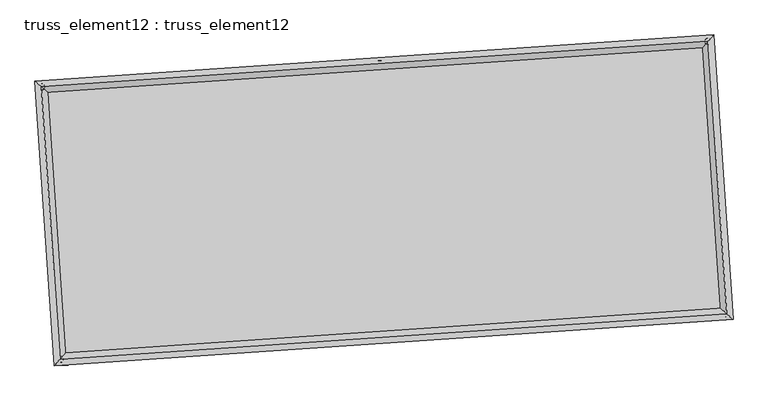
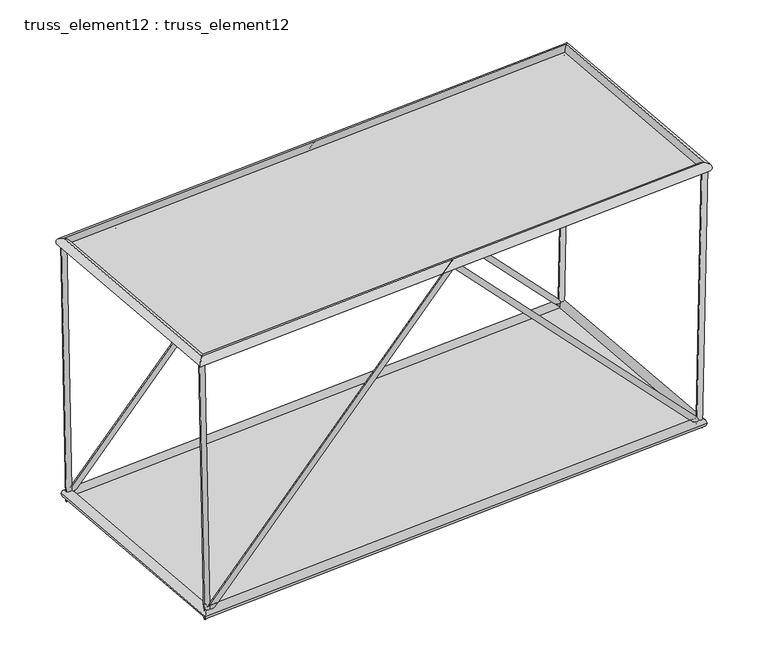
"""IFC4 building model written with IfcOpenShell, lengths in millimetres: plate geometry, truss_element12 : truss_element12."""

import ifcopenshell
import ifcopenshell.guid

model = None  # the IFC model being written
_history = None  # IfcOwnerHistory: only IFC2X3 demands one
_inside = {}  # id of a spatial element -> (the spatial element, [elements in it])
_under = {}  # id of a project, library or spatial element -> (it, [spatial elements below it])
_declared = {}  # id of a project -> (the project, [libraries it declares])
_typed = {}  # id of a type object -> (the type object, [elements of that type])
_made_of = {}  # id of a material, layer set ... -> (it, [elements and type objects made of it])


def new_model(schema):
    """Start an empty IFC model of exactly this schema.

    Asked for "IFC4X3", IfcOpenShell would pick the latest addendum, in which some entities
    have other attributes; the version numbers below select the first issue.
    IFC2X3 requires an IfcOwnerHistory on every rooted entity: one is made here for all.
    """
    global model, _history
    if schema == "IFC4X3":
        model = ifcopenshell.file(schema_version=(4, 3, 0, 0))
    else:
        model = ifcopenshell.file(schema=schema)
    _inside.clear()
    _under.clear()
    _declared.clear()
    _typed.clear()
    _made_of.clear()
    _history = None
    if model.schema == "IFC2X3":
        org = make("IfcOrganization", Name="unknown")
        user = make(
            "IfcPersonAndOrganization",
            ThePerson=make("IfcPerson", FamilyName="unknown"),
            TheOrganization=org,
        )
        app = make(
            "IfcApplication",
            ApplicationDeveloper=org,
            Version="unknown",
            ApplicationFullName="unknown",
            ApplicationIdentifier="unknown",
        )
        _history = make(
            "IfcOwnerHistory",
            OwningUser=user,
            OwningApplication=app,
            ChangeAction="ADDED",
            CreationDate=0,
        )
    return model


def make(cls, **values):
    """One entity of the class cls with the attributes given. An attribute that is None is left unset."""
    return model.create_entity(
        cls, **{name: value for name, value in values.items() if value is not None}
    )


def rooted(cls, **values):
    """An entity with a GlobalId (a new one), such as an element, a storey or a relation."""
    return make(cls, GlobalId=ifcopenshell.guid.new(), OwnerHistory=_history, **values)


def si_unit(unit_type, name, prefix=None):
    """IfcSIUnit, for example si_unit("LENGTHUNIT", "METRE", prefix="MILLI")."""
    return make("IfcSIUnit", UnitType=unit_type, Prefix=prefix, Name=name)


def assignment(units):
    """IfcUnitAssignment: the units of a project."""
    return None if units is None else make("IfcUnitAssignment", Units=units)


def point(xyz):
    """IfcCartesianPoint."""
    return None if xyz is None else make("IfcCartesianPoint", Coordinates=xyz)


def direction(xyz):
    """IfcDirection."""
    return None if xyz is None else make("IfcDirection", DirectionRatios=xyz)


def frame(location, z_axis=None, x_axis=None):
    """IfcAxis2Placement3D, a coordinate frame: its origin and axes. An axis left out is left unset."""
    return make(
        "IfcAxis2Placement3D",
        Location=point(location),
        Axis=direction(z_axis),
        RefDirection=direction(x_axis),
    )


def origin():
    """The frame at (0, 0, 0) with its axes left unset."""
    return frame((0.0, 0.0, 0.0))


def origin_with_axes():
    """The frame at (0, 0, 0) with the z axis (0, 0, 1) and the x axis (1, 0, 0) written out."""
    return frame((0.0, 0.0, 0.0), z_axis=(0.0, 0.0, 1.0), x_axis=(1.0, 0.0, 0.0))


def place(relative_to, where):
    """IfcLocalPlacement: puts the frame where relative to a parent placement (None: the world)."""
    return make(
        "IfcLocalPlacement", PlacementRelTo=relative_to, RelativePlacement=where
    )


def context(
    kind, dimensions, precision=None, world=None, true_north=None, identifier=None
):
    """IfcGeometricRepresentationContext, for example the 3D "Model" context."""
    return make(
        "IfcGeometricRepresentationContext",
        ContextIdentifier=identifier,
        ContextType=kind,
        CoordinateSpaceDimension=dimensions,
        Precision=precision,
        WorldCoordinateSystem=world,
        TrueNorth=true_north,
    )


def project(units=None, contexts=None):
    """IfcProject with its units and contexts."""
    return rooted(
        "IfcProject",
        Name="project",
        RepresentationContexts=contexts,
        UnitsInContext=assignment(units),
    )


def spatial(cls, under=None, at=None, **own):
    """A site, building, storey or space (cls), placed at a placement, below another one or the project."""
    s = rooted(cls, ObjectPlacement=at, **own)
    if under is not None:
        _under.setdefault(under.id(), (under, []))[1].append(s)
    return s


def polyline(points):
    """IfcPolyline through the points."""
    return make("IfcPolyline", Points=[point(p) for p in points])


def circle_curve(where, radius):
    """IfcCircle in the frame where."""
    return make("IfcCircle", Position=where, Radius=radius)


def ellipse_curve(where, semi_axis1, semi_axis2):
    """IfcEllipse in the frame where."""
    return make(
        "IfcEllipse", Position=where, SemiAxis1=semi_axis1, SemiAxis2=semi_axis2
    )


def outline(outer, holes=None, kind="AREA"):
    """IfcArbitraryClosedProfileDef: a profile drawn as a closed curve; with holes, ...WithVoids."""
    if holes is None:
        return make("IfcArbitraryClosedProfileDef", ProfileType=kind, OuterCurve=outer)
    return make(
        "IfcArbitraryProfileDefWithVoids",
        ProfileType=kind,
        OuterCurve=outer,
        InnerCurves=holes,
    )


def extrude(swept, where, along, depth):
    """IfcExtrudedAreaSolid: the profile swept, set in the frame where, extruded along a direction by depth."""
    return make(
        "IfcExtrudedAreaSolid",
        SweptArea=swept,
        Position=where,
        ExtrudedDirection=direction(along),
        Depth=depth,
    )


def shape(context_of_items, identifier, shape_type, items):
    """IfcShapeRepresentation: the items that make up one representation, for example the "Body"."""
    return make(
        "IfcShapeRepresentation",
        ContextOfItems=context_of_items,
        RepresentationIdentifier=identifier,
        RepresentationType=shape_type,
        Items=items,
    )


def source(mapping_origin, context_of_items, identifier, shape_type, items):
    """IfcRepresentationMap: a shape defined once, which mapped items show again and again."""
    return make(
        "IfcRepresentationMap",
        MappingOrigin=mapping_origin,
        MappedRepresentation=shape(context_of_items, identifier, shape_type, items),
    )


def transform(
    local_origin,
    x_axis=None,
    y_axis=None,
    z_axis=None,
    scale=None,
    scale2=None,
    scale3=None,
    uniform=True,
):
    """IfcCartesianTransformationOperator3D, or its non-uniform kind. x_axis, y_axis, z_axis: its Axis1, 2, 3."""
    if uniform:
        return make(
            "IfcCartesianTransformationOperator3D",
            Axis1=direction(x_axis),
            Axis2=direction(y_axis),
            LocalOrigin=point(local_origin),
            Scale=scale,
            Axis3=direction(z_axis),
        )
    return make(
        "IfcCartesianTransformationOperator3DnonUniform",
        Axis1=direction(x_axis),
        Axis2=direction(y_axis),
        LocalOrigin=point(local_origin),
        Scale=scale,
        Axis3=direction(z_axis),
        Scale2=scale2,
        Scale3=scale3,
    )


def mapped(mapping_source, mapping_target):
    """IfcMappedItem: shows the shape of a source again, moved by a transform."""
    return make(
        "IfcMappedItem", MappingSource=mapping_source, MappingTarget=mapping_target
    )


def made_of(thing, what):
    """Note that an element or type object is made of a material, layer set ...; save() writes the relation."""
    if what is not None:
        _made_of.setdefault(what.id(), (what, []))[1].append(thing)
    return thing


def element(
    cls,
    number,
    at=None,
    inside=None,
    cuts=None,
    type_object=None,
    material=None,
    context=None,
    identifier="Body",
    shape_type=None,
    held_by="IfcProductDefinitionShape",
    body=None,
    shapes=None,
    **own,
):
    """One element of the class cls, such as IfcWall. Its Tag is "e" and its number.

    at: its placement. inside: the storey or other place that contains it. cuts: it is an
    opening in that element (IfcRelVoidsElement). A single representation is given by context,
    identifier, shape_type and body (its items); several are given by shapes. held_by: the class
    of the entity that holds the representations. save() writes the other relations.
    """
    e = rooted(cls, Tag="e%d" % number, ObjectPlacement=at, **own)
    if body is not None:
        shapes = [shape(context, identifier, shape_type, body)]
    if shapes is not None:
        e.Representation = make(held_by, Representations=shapes)
    if inside is not None:
        _inside.setdefault(inside.id(), (inside, []))[1].append(e)
    if cuts is not None:
        rooted(
            "IfcRelVoidsElement", RelatingBuildingElement=cuts, RelatedOpeningElement=e
        )
    if type_object is not None:
        _typed.setdefault(type_object.id(), (type_object, []))[1].append(e)
    return made_of(e, material)


def aggregate(whole, parts):
    """IfcRelAggregates: a whole, such as a stair, and the parts it consists of."""
    return rooted("IfcRelAggregates", RelatingObject=whole, RelatedObjects=parts)


def save(model, path):
    """Write the relations noted so far, then the file.

    IfcRelAggregates (storeys below a building ...), IfcRelContainedInSpatialStructure (elements
    in a storey), IfcRelDefinesByType, IfcRelAssociatesMaterial and IfcRelDeclares: one each for
    every whole, place, type object, material and project.
    """
    for whole, parts in _under.values():
        aggregate(whole, parts)
    for where, things in _inside.values():
        rooted(
            "IfcRelContainedInSpatialStructure",
            RelatedElements=things,
            RelatingStructure=where,
        )
    for kind, things in _typed.values():
        rooted("IfcRelDefinesByType", RelatedObjects=things, RelatingType=kind)
    for what, things in _made_of.values():
        rooted("IfcRelAssociatesMaterial", RelatedObjects=things, RelatingMaterial=what)
    for by, libraries in _declared.values():
        rooted("IfcRelDeclares", RelatingContext=by, RelatedDefinitions=libraries)
    model.write(path)


def plane_surface(at):
    """IfcPlane: the flat surface through the origin of the frame at, square to its z axis."""
    return make("IfcPlane", Position=at)


def cylinder_surface(at, radius):
    """IfcCylindricalSurface: all points at the distance radius from the z axis of the frame at."""
    return make("IfcCylindricalSurface", Position=at, Radius=radius)


def advanced_brep(points, edges, surfaces, faces):
    """IfcAdvancedBrep: a solid bounded by faces that lie on surfaces and meet in shared edges.

    An edge is (start, end): straight between two places in points (the first is 0);
    or (start, end, curve); or (start, end, curve, False) where it runs against its curve.
    A face is (place in surfaces, loops), or (place, loops, False) where it looks against
    its surface's normal. A loop lists edges by number (the first is 1), with a minus sign
    where the edge is run from its end to its start. The first loop is the outer one.
    """
    corners = [point(p) for p in points]
    vertices = [make("IfcVertexPoint", VertexGeometry=c) for c in corners]
    made = []
    for start, end, *more in edges:
        made.append(
            make(
                "IfcEdgeCurve",
                EdgeStart=vertices[start],
                EdgeEnd=vertices[end],
                EdgeGeometry=more[0] if more else make("IfcPolyline", Points=[corners[start], corners[end]]),
                SameSense=more[1] if len(more) > 1 else True,
            )
        )
    hull = []
    for where, loops, *sense in faces:
        bounds = []
        for j, loop in enumerate(loops):
            ring = [make("IfcOrientedEdge", EdgeElement=made[abs(k) - 1], Orientation=k > 0) for k in loop]
            bounds.append(
                make(
                    "IfcFaceOuterBound" if j == 0 else "IfcFaceBound",
                    Bound=make("IfcEdgeLoop", EdgeList=ring),
                    Orientation=True,
                )
            )
        hull.append(make("IfcAdvancedFace", Bounds=bounds, FaceSurface=surfaces[where], SameSense=sense[0] if sense else True))
    return make("IfcAdvancedBrep", Outer=make("IfcClosedShell", CfsFaces=hull))


def truss_element12_truss_element12_2df4d8d8(model_context):
    return source(origin(), model_context, "Body", "SolidModel", [
        advanced_brep(
        [(-3764.5300605, 2269.433423, 4999.9996325), (-3863.6135877, 2256.0735143, 4998.0077777), (-3667.3556051, 2276.0593798, 121.6771544), (-3761.6312777, 2263.0273003, -121.6771544), (1063.0371685, 2598.6068811, 5071.1337274), (1063.495558, 2592.0343572, 4926.9006014), (5794.7619233, 2921.2452051, 121.686477), (5889.9990537, 2921.1352834, -121.686477), (5890.6143162, 2927.7810154, 5000.0130059), (5990.5947849, 2927.9945239, 4998.0482415)],
        [
            (0, 1, circle_curve(frame((-3814.0718241, 2262.7534687, 4999.0037051), z_axis=(-0.019915676532372622, -0.001357974276168432, 0.9998007410149901), x_axis=(-0.13359951548632418, 0.9910345300462156, -0.001315187399616253)), 50.0)),
            (1, 0, circle_curve(frame((-3814.0718241, 2262.7534687, 4999.0037051), z_axis=(-0.019915676532372622, -0.001357974276168432, 0.9998007410149901), x_axis=(-0.13359951548632418, 0.9910345300462156, -0.001315187399616253)), 50.0)),
            (0, 2),
            (2, 3, ellipse_curve(frame((-3714.4934414, 2269.54334, 0.0), z_axis=(-0.9294501915680613, -0.06337567539207484, 0.36346370542695533), x_axis=(0.36262170398032334, 0.024725795540271416, 0.9316083591495449)), 130.8941732, 50.0)),
            (3, 1),
            (3, 2, ellipse_curve(frame((-3714.4934414, 2269.54334, 0.0), z_axis=(-0.9294501915680613, -0.06337567539207484, 0.36346370542695533), x_axis=(0.36262170398032334, 0.024725795540271416, 0.9316083591495449)), 130.8941732, 50.0)),
            (2, 4),
            (4, 5, ellipse_curve(frame((1063.2663632, 2595.3206192, 4999.0171644), z_axis=(-0.9976833935750009, -0.06802823805824446, -7.079096398268556e-05), x_axis=(7.062696935752604e-05, 4.815784562388573e-06, -0.9999999974943197)), 72.2735967, 50.0)),
            (5, 3),
            (5, 4, ellipse_curve(frame((1063.2663632, 2595.3206192, 4999.0171644), z_axis=(-0.9976833935750009, -0.06802823805824446, -7.079096398268556e-05), x_axis=(7.062696935752604e-05, 4.815784562388573e-06, -0.9999999974943197)), 72.2735967, 50.0)),
            (4, 6),
            (6, 7, ellipse_curve(frame((5842.3804885, 2921.1902443, 0.0), z_axis=(-0.929375267082314, -0.06337056657620659, -0.36365613459350316), x_axis=(-0.3628136873647087, -0.024738886157455623, 0.9315332606904125)), 130.9147553, 50.0)),
            (7, 5),
            (7, 6, ellipse_curve(frame((5842.3804885, 2921.1902443, 0.0), z_axis=(-0.929375267082314, -0.06337056657620659, -0.36365613459350316), x_axis=(-0.3628136873647087, -0.024738886157455623, 0.9315332606904125)), 130.9147553, 50.0)),
            (8, 9, circle_curve(frame((5940.6045505, 2927.8877697, 4999.0306237), z_axis=(0.019644812406203346, 0.0013395050810558434, 0.9998061247420236), x_axis=(-0.0021609883682618125, 0.9999968235657783, -0.001297300129496852)), 50.0)),
            (9, 8, circle_curve(frame((5940.6045505, 2927.8877697, 4999.0306237), z_axis=(0.019644812406203346, 0.0013395050810558434, 0.9998061247420236), x_axis=(-0.0021609883682618125, 0.9999968235657783, -0.001297300129496852)), 50.0)),
            (6, 8),
            (9, 7),
        ],
        [
            plane_surface(frame((-3814.0718241, 2312.7534225, 4999.0716173), z_axis=(-0.019915676532371102, -0.001357974276169366, 0.9998007410149901), x_axis=(0.9998016632453949, -2.7050341500078914e-05, 0.01991565816188513))),
            cylinder_surface(frame((-3814.0718241, 2262.7534687, 4999.0037051), z_axis=(-0.019915676532372622, -0.001357974276168432, 0.9998007410149901), x_axis=(-0.13359951548632418, 0.9910345300462156, -0.001315187399616253)), 50.0),
            cylinder_surface(frame((-3714.4934414, 2269.54334, 0.0), z_axis=(-0.6901619145465996, -0.04705951740188029, -0.7221232121537671), x_axis=(-0.020413692768052043, 0.9987522410377818, -0.045576772259345893)), 50.0),
            cylinder_surface(frame((1063.2663632, 2595.3206192, 4999.0171644), z_axis=(-0.6902639103769979, -0.04706647210983291, 0.722025263570597), x_axis=(-0.11534072659634662, 0.9922795274524686, -0.0455835078392663)), 50.0),
            plane_surface(frame((5940.6045505, 2877.8878145, 4999.0976119), z_axis=(0.01964481240620162, 0.001339505081055023, 0.9998061247420239), x_axis=(0.9998070220525186, -2.631940509978392e-05, -0.0196447947753029))),
            cylinder_surface(frame((5842.3804885, 2921.1902443, 0.0), z_axis=(-0.01964481240620335, -0.0013395050810558436, -0.9998061247420238), x_axis=(-0.0021609883682618125, 0.9999968235657783, -0.001297300129496852)), 50.0),
        ],
        [
            (0, [[1, 2]]),
            (1, [[-1, 3, 4, 5]]),
            (1, [[-2, -5, 6, -3]]),
            (2, [[-4, 7, 8, 9]]),
            (2, [[-6, -9, 10, -7]]),
            (3, [[-8, 11, 12, 13]]),
            (3, [[-10, -13, 14, -11]]),
            (4, [[15, 16]]),
            (5, [[-12, 17, -16, 18]]),
            (5, [[-14, -18, -15, -17]]),
        ],
    ),
        advanced_brep(
        [(-3492.4171076, -1721.3001613, 4999.9996325), (-3591.5006347, -1734.66007, 4998.0077777), (-3395.2426522, -1714.6742045, 121.6771544), (-3489.5183248, -1727.706284, -121.6771544), (1335.1501214, -1392.1267032, 5071.1337274), (1335.6085109, -1398.6992271, 4926.9006014), (6066.8748762, -1069.4883792, 121.686477), (6162.1120066, -1069.5983009, -121.686477), (6162.7272691, -1062.9525689, 5000.0130059), (6262.7077378, -1062.7390604, 4998.0482415)],
        [
            (0, 1, circle_curve(frame((-3541.9588712, -1727.9801156, 4999.0037051), z_axis=(-0.019915676532372775, -0.001357974276168436, 0.9998007410149901), x_axis=(-0.13359951548632507, 0.9910345300462154, -0.001315187399616287)), 50.0)),
            (1, 0, circle_curve(frame((-3541.9588712, -1727.9801156, 4999.0037051), z_axis=(-0.019915676532372775, -0.001357974276168436, 0.9998007410149901), x_axis=(-0.13359951548632507, 0.9910345300462154, -0.001315187399616287)), 50.0)),
            (0, 2),
            (2, 3, ellipse_curve(frame((-3442.3804885, -1721.1902443, 0.0), z_axis=(-0.9294501915680613, -0.06337567539207523, 0.36346370542695516), x_axis=(0.3626217039803232, 0.024725795540271572, 0.9316083591495451)), 130.8941732, 50.0)),
            (3, 1),
            (3, 2, ellipse_curve(frame((-3442.3804885, -1721.1902443, 0.0), z_axis=(-0.9294501915680613, -0.06337567539207523, 0.36346370542695516), x_axis=(0.3626217039803232, 0.024725795540271572, 0.9316083591495451)), 130.8941732, 50.0)),
            (2, 4),
            (4, 5, ellipse_curve(frame((1335.3793161, -1395.4129651, 4999.0171644), z_axis=(-0.9976833935750009, -0.0680282380582447, -7.079096398276582e-05), x_axis=(7.062696935767979e-05, 4.815784562205989e-06, -0.9999999974943197)), 72.2735967, 50.0)),
            (5, 3),
            (5, 4, ellipse_curve(frame((1335.3793161, -1395.4129651, 4999.0171644), z_axis=(-0.9976833935750009, -0.0680282380582447, -7.079096398276582e-05), x_axis=(7.062696935767979e-05, 4.815784562205989e-06, -0.9999999974943197)), 72.2735967, 50.0)),
            (4, 6),
            (6, 7, ellipse_curve(frame((6114.4934414, -1069.54334, 0.0), z_axis=(-0.9293752670823138, -0.06337056657620667, -0.36365613459350354), x_axis=(-0.3628136873647092, -0.02473888615745564, 0.9315332606904123)), 130.9147553, 50.0)),
            (7, 5),
            (7, 6, ellipse_curve(frame((6114.4934414, -1069.54334, 0.0), z_axis=(-0.9293752670823138, -0.06337056657620667, -0.36365613459350354), x_axis=(-0.3628136873647092, -0.02473888615745564, 0.9315332606904123)), 130.9147553, 50.0)),
            (8, 9, circle_curve(frame((6212.7175034, -1062.8458146, 4999.0306237), z_axis=(0.019644812406202576, 0.0013395050810558389, 0.9998061247420237), x_axis=(-0.002160988368261633, 0.9999968235657782, -0.0012973001294968524)), 50.0)),
            (9, 8, circle_curve(frame((6212.7175034, -1062.8458146, 4999.0306237), z_axis=(0.019644812406202576, 0.0013395050810558389, 0.9998061247420237), x_axis=(-0.002160988368261633, 0.9999968235657782, -0.0012973001294968524)), 50.0)),
            (6, 8),
            (9, 7),
        ],
        [
            plane_surface(frame((-3541.9588712, -1677.9801618, 4999.0716173), z_axis=(-0.019915676532374655, -0.0013579742761693696, 0.99980074101499), x_axis=(0.9998016632453948, -2.7050341500078914e-05, 0.019915658161888682))),
            cylinder_surface(frame((-3541.9588712, -1727.9801156, 4999.0037051), z_axis=(-0.019915676532372775, -0.001357974276168436, 0.9998007410149901), x_axis=(-0.13359951548632507, 0.9910345300462154, -0.001315187399616287)), 50.0),
            cylinder_surface(frame((-3442.3804885, -1721.1902443, 0.0), z_axis=(-0.6901619145465994, -0.047059517401880586, -0.7221232121537672), x_axis=(-0.02041369276805217, 0.9987522410377818, -0.04557677225934618)), 50.0),
            cylinder_surface(frame((1335.3793161, -1395.4129651, 4999.0171644), z_axis=(-0.690263910376998, -0.04706647210983294, 0.722025263570597), x_axis=(-0.115340726596347, 0.9922795274524685, -0.04558350783926664)), 50.0),
            plane_surface(frame((6212.7175034, -1112.8457698, 4999.0976119), z_axis=(0.019644812406201615, 0.0013395050810550285, 0.9998061247420239), x_axis=(0.9998070220525186, -2.6319405099339832e-05, -0.0196447947753029))),
            cylinder_surface(frame((6114.4934414, -1069.54334, 0.0), z_axis=(-0.019644812406202576, -0.0013395050810558389, -0.9998061247420237), x_axis=(-0.002160988368261633, 0.9999968235657782, -0.0012973001294968524)), 50.0),
        ],
        [
            (0, [[1, 2]]),
            (1, [[-1, 3, 4, 5]]),
            (1, [[-2, -5, 6, -3]]),
            (2, [[-4, 7, 8, 9]]),
            (2, [[-6, -9, 10, -7]]),
            (3, [[-8, 11, 12, 13]]),
            (3, [[-10, -13, 14, -11]]),
            (4, [[15, 16]]),
            (5, [[-12, 17, -16, 18]]),
            (5, [[-14, -18, -15, -17]]),
        ],
    ),
        advanced_brep(
        [(-3541.9518595, -1727.9723443, 4909.0037054), (-3541.9658829, -1727.987887, 5089.0037048), (-3814.0798258, 2262.7602163, 5089.0037048), (-3814.0638224, 2262.746721, 4909.0037054), (5940.6110678, 2927.8955073, 5089.0306234), (5940.5980333, 2927.880032, 4909.030624), (6212.7250107, -1062.852596, 5089.0306234), (6212.7099962, -1062.8390333, 4909.030624)],
        [
            (0, 1, ellipse_curve(frame((-3541.9588712, -1727.9801156, 4999.0037051), z_axis=(-0.7535719234027851, 0.657365466278262, -1.9467846691616333e-06), x_axis=(-0.6573654662754057, -0.7535719234052768, -1.9467846691616053e-06)), 127.2792206, 90.0)),
            (1, 2),
            (2, 3, ellipse_curve(frame((-3814.0718241, 2262.7534687, 4999.0037051), z_axis=(-0.657365466275406, -0.7535719234052765, -1.946784669239898e-06), x_axis=(0.7535719234027848, -0.6573654662782622, 1.946784669239924e-06)), 127.2792206, 90.0)),
            (3, 0),
            (1, 0, ellipse_curve(frame((-3541.9588712, -1727.9801156, 4999.0037051), z_axis=(-0.7535719234027851, 0.657365466278262, -1.9467846691616333e-06), x_axis=(-0.6573654662754057, -0.7535719234052768, -1.9467846691616053e-06)), 127.2792206, 90.0)),
            (3, 2, ellipse_curve(frame((-3814.0718241, 2262.7534687, 4999.0037051), z_axis=(-0.657365466275406, -0.7535719234052765, -1.946784669239898e-06), x_axis=(0.7535719234027848, -0.6573654662782622, 1.946784669239924e-06)), 127.2792206, 90.0)),
            (2, 4),
            (4, 5, ellipse_curve(frame((5940.6045505, 2927.8877697, 4999.0306237), z_axis=(-0.7535719234027848, 0.6573654662782625, -1.946784669048477e-06), x_axis=(-0.6573654662754064, -0.7535719234052762, -1.9467846694313455e-06)), 127.2792206, 90.0)),
            (5, 3),
            (5, 4, ellipse_curve(frame((5940.6045505, 2927.8877697, 4999.0306237), z_axis=(-0.7535719234027848, 0.6573654662782625, -1.946784669048477e-06), x_axis=(-0.6573654662754064, -0.7535719234052762, -1.9467846694313455e-06)), 127.2792206, 90.0)),
            (4, 6),
            (6, 7, ellipse_curve(frame((6212.7175034, -1062.8458146, 4999.0306237), z_axis=(0.6573654662754065, 0.7535719234052762, 1.9467846693530547e-06), x_axis=(-0.7535719234027849, 0.6573654662782625, -1.946784668970186e-06)), 127.2792206, 90.0)),
            (7, 5),
            (7, 6, ellipse_curve(frame((6212.7175034, -1062.8458146, 4999.0306237), z_axis=(0.6573654662754065, 0.7535719234052762, 1.9467846693530547e-06), x_axis=(-0.7535719234027849, 0.6573654662782625, -1.946784668970186e-06)), 127.2792206, 90.0)),
            (6, 1),
            (0, 7),
        ],
        [
            cylinder_surface(frame((-3541.9588712, -1727.9801156, 4999.0037051), z_axis=(0.06802823822870271, -0.9976833960748768, 0.0), x_axis=(-0.9976833925883778, -0.0680282379909716, -8.36013684286445e-05)), 90.0),
            cylinder_surface(frame((-3814.0718241, 2262.7534687, 4999.0037051), z_axis=(-0.9976833960710954, -0.06802823822844452, -2.7531692822591026e-06), x_axis=(-0.06802823778429826, 0.9976833928293743, -8.08481991553833e-05)), 90.0),
            cylinder_surface(frame((5940.6045505, 2927.8877697, 4999.0306237), z_axis=(-0.06802823822870169, 0.9976833960748768, 0.0), x_axis=(0.9976833930325241, 0.06802823802125522, -7.809502988239287e-05)), 90.0),
            cylinder_surface(frame((6212.7175034, -1062.8458146, 4999.0306237), z_axis=(0.9976833960710954, 0.06802823822844468, 2.753169282148382e-06), x_axis=(0.06802823822844468, -0.9976833927990898, -8.084819915581397e-05)), 90.0),
        ],
        [
            (0, [[1, 2, 3, 4]]),
            (0, [[5, -4, 6, -2]]),
            (1, [[-3, 7, 8, 9]]),
            (1, [[-6, -9, 10, -7]]),
            (2, [[-8, 11, 12, 13]]),
            (2, [[-10, -13, 14, -11]]),
            (3, [[-12, 15, -1, 16]]),
            (3, [[-14, -16, -5, -15]]),
        ],
    ),
        advanced_brep(
        [(-3358.7115243, -1625.2761972, 0.0), (-3526.0494527, -1817.1042913, 0.0), (-3810.4074885, 2353.2123043, 0.0), (-3618.5793943, 2185.8743758, 0.0), (5926.0494527, 3017.1042913, 0.0), (5758.7115243, 2825.2761972, 0.0), (6210.4074885, -1153.2123043, 0.0), (6018.5793943, -985.8743758, 0.0)],
        [
            (0, 1, ellipse_curve(frame((-3442.3804885, -1721.1902443, 0.0), z_axis=(-0.7535719234054582, 0.6573654662780805, 0.0), x_axis=(-0.6573654662780805, -0.7535719234054584, 0.0)), 127.2792206, 90.0)),
            (1, 2),
            (2, 3, ellipse_curve(frame((-3714.4934414, 2269.54334, 0.0), z_axis=(-0.6573654662780806, -0.7535719234054582, 0.0), x_axis=(0.7535719234054582, -0.6573654662780803, 0.0)), 127.2792206, 90.0)),
            (3, 0),
            (1, 0, ellipse_curve(frame((-3442.3804885, -1721.1902443, 0.0), z_axis=(-0.7535719234054582, 0.6573654662780805, 0.0), x_axis=(-0.6573654662780805, -0.7535719234054584, 0.0)), 127.2792206, 90.0)),
            (3, 2, ellipse_curve(frame((-3714.4934414, 2269.54334, 0.0), z_axis=(-0.6573654662780806, -0.7535719234054582, 0.0), x_axis=(0.7535719234054582, -0.6573654662780803, 0.0)), 127.2792206, 90.0)),
            (2, 4),
            (4, 5, ellipse_curve(frame((5842.3804885, 2921.1902443, 0.0), z_axis=(-0.7535719234054578, 0.657365466278081, 0.0), x_axis=(-0.6573654662780812, -0.7535719234054578, 0.0)), 127.2792206, 90.0)),
            (5, 3),
            (5, 4, ellipse_curve(frame((5842.3804885, 2921.1902443, 0.0), z_axis=(-0.7535719234054578, 0.657365466278081, 0.0), x_axis=(-0.6573654662780812, -0.7535719234054578, 0.0)), 127.2792206, 90.0)),
            (4, 6),
            (6, 7, ellipse_curve(frame((6114.4934414, -1069.54334, 0.0), z_axis=(0.657365466278081, 0.7535719234054578, 0.0), x_axis=(-0.7535719234054578, 0.657365466278081, 0.0)), 127.2792206, 90.0)),
            (7, 5),
            (7, 6, ellipse_curve(frame((6114.4934414, -1069.54334, 0.0), z_axis=(0.657365466278081, 0.7535719234054578, 0.0), x_axis=(-0.7535719234054578, 0.657365466278081, 0.0)), 127.2792206, 90.0)),
            (6, 1),
            (0, 7),
        ],
        [
            cylinder_surface(frame((-3442.3804885, -1721.1902443, 0.0), z_axis=(0.06802823822870181, -0.9976833960748765, 0.0), x_axis=(-0.9976833960748765, -0.06802823822870181, 0.0)), 90.0),
            cylinder_surface(frame((-3714.4934414, 2269.54334, 0.0), z_axis=(-0.9976833960748767, -0.06802823822870133, 0.0), x_axis=(-0.06802823822870133, 0.9976833960748767, 0.0)), 90.0),
            cylinder_surface(frame((5842.3804885, 2921.1902443, 0.0), z_axis=(-0.06802823822870059, 0.9976833960748768, 0.0), x_axis=(0.9976833960748768, 0.06802823822870059, 0.0)), 90.0),
            cylinder_surface(frame((6114.4934414, -1069.54334, 0.0), z_axis=(0.9976833960748768, 0.06802823822870133, 0.0), x_axis=(0.06802823822870133, -0.9976833960748768, 0.0)), 90.0),
        ],
        [
            (0, [[1, 2, 3, 4]]),
            (0, [[5, -4, 6, -2]]),
            (1, [[-3, 7, 8, 9]]),
            (1, [[-6, -9, 10, -7]]),
            (2, [[-8, 11, 12, 13]]),
            (2, [[-10, -13, 14, -11]]),
            (3, [[-12, 15, -1, 16]]),
            (3, [[-14, -16, -5, -15]]),
        ],
    ),
        extrude(outline(polyline([(-3442.3804885, -1721.1902443), (-3714.4934414, 2269.54334), (5842.3804885, 2921.1902443), (6114.4934414, -1069.54334), (-3442.3804885, -1721.1902443)])), origin_with_axes(), (0.0, 0.0, 1.0), 20.0),
        extrude(outline(polyline([(-2000.0, 4888.6632839), (2000.0, 4888.6632839), (2000.0000001, -4888.6632838), (-1999.9999999, -4888.6632838), (-2000.0, 4888.6632839)])), frame((1199.3228397, 599.953827, 4999.0171644), z_axis=(-2.7467912794933064e-06, -1.8729325581746698e-07, 0.9999999999962101), x_axis=(-0.06802823822870173, 0.9976833960748767, 0.0)), (0.0, 0.0, 1.0), 20.0),
    ])


if __name__ == "__main__":
    model = new_model("IFC4")
    model_context = context("Model", 3, world=origin())
    ifc_project = project(units=[si_unit("LENGTHUNIT", "METRE", prefix="MILLI")], contexts=[model_context])
    site = spatial("IfcSite", under=ifc_project)
    building = spatial("IfcBuilding", under=site)
    placement = place(None, origin())
    truss_element12_truss_element12_shape = truss_element12_truss_element12_2df4d8d8(model_context)
    element("IfcPlate", 1, ObjectType="truss_element12 : truss_element12", at=placement, inside=building, context=model_context, shape_type="MappedRepresentation", body=[
        mapped(truss_element12_truss_element12_shape, transform((0.0, 0.0, 0.0), x_axis=(1.0, 0.0, 0.0), y_axis=(0.0, 1.0, 0.0), z_axis=(0.0, 0.0, 1.0))),
    ])
    save(model, "model.ifc")

# Revit data of these elements
# Type "truss_element12 : truss_element12"
#   steellbar1 = 90 mm
#   steelbar2 = 50 mm
#   offset1 = 5000 mm
#   M = Default Roof
# Element 1 (IfcPlate, "truss_element12 : truss_element12")
#   Materials on its faces: "Default Roof"
# Materials
#   "Default Roof": class "Miscellaneous", colour RGB 0 127 0, transparency 0, Comments = "Rendering appearance not upgraded Rendering appearance not upgraded ", Cost = 0
